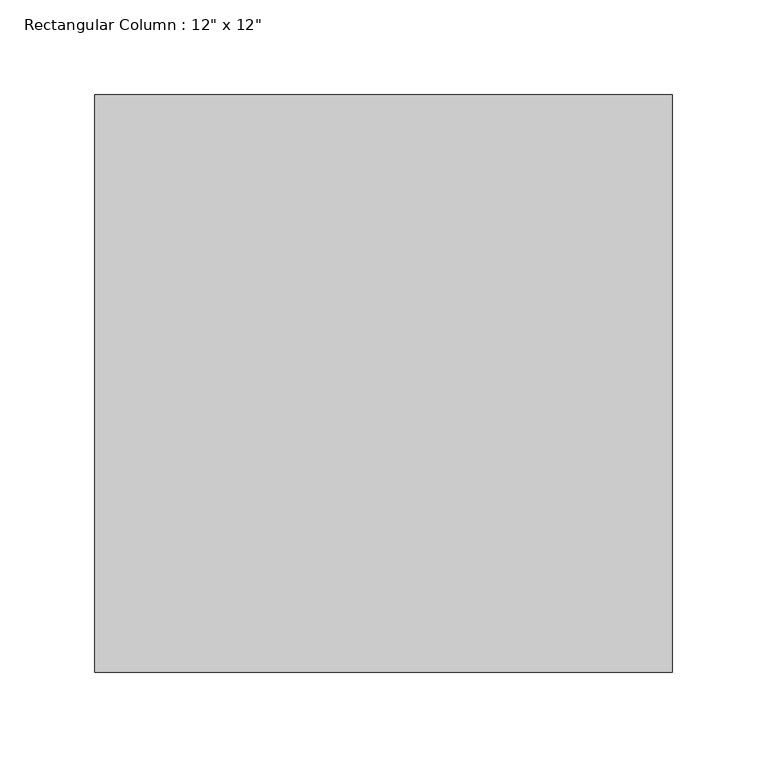
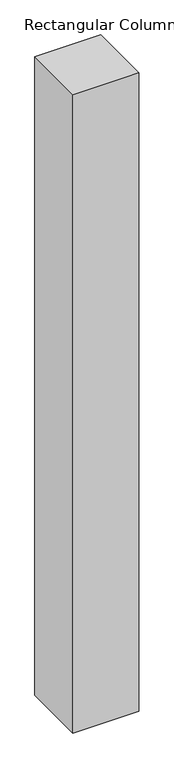
"""IFC4 building model written with IfcOpenShell, lengths in millimetres: column geometry."""

from ifc_helpers import new_model, si_unit, frame, origin, place, context, project, spatial, polyline, outline, extrude, source, transform, mapped, element, save


def column_96c5ed10(model_context):
    return source(origin(), model_context, "Body", "SweptSolid", [
        extrude(outline(polyline([(152.4, 152.4), (152.4, -152.4), (-152.4, -152.4), (-152.4, 152.4), (152.4, 152.4)])), frame((0.0, 0.0, -381.0), z_axis=(0.0, 0.0, 1.0), x_axis=(1.0, 0.0, 0.0)), (0.0, 0.0, 1.0), 3124.2),
    ])


if __name__ == "__main__":
    model = new_model("IFC4")
    model_context = context("Model", 3, world=origin())
    ifc_project = project(units=[si_unit("LENGTHUNIT", "METRE", prefix="MILLI")], contexts=[model_context])
    site = spatial("IfcSite", under=ifc_project)
    building = spatial("IfcBuilding", under=site)
    placement = place(None, origin())
    column_shape = column_96c5ed10(model_context)
    element("IfcColumn", 1, ObjectType="Rectangular Column : 12\" x 12\"", at=placement, inside=building, context=model_context, shape_type="MappedRepresentation", body=[
        mapped(column_shape, transform((0.0, 0.0, 0.0), x_axis=(1.0, 0.0, 0.0), y_axis=(0.0, 1.0, 0.0), z_axis=(0.0, 0.0, 1.0))),
    ])
    save(model, "model.ifc")

# Revit data of these elements
# Type "Rectangular Column : 12\" x 12\""
#   Assembly Code = "B1010200"
#   Depth = 1' - 0"
#   Offset Base = 0' - 0"
#   Offset Top = 0' - 0"
#   Width = 1' - 0"
#   Material = none
